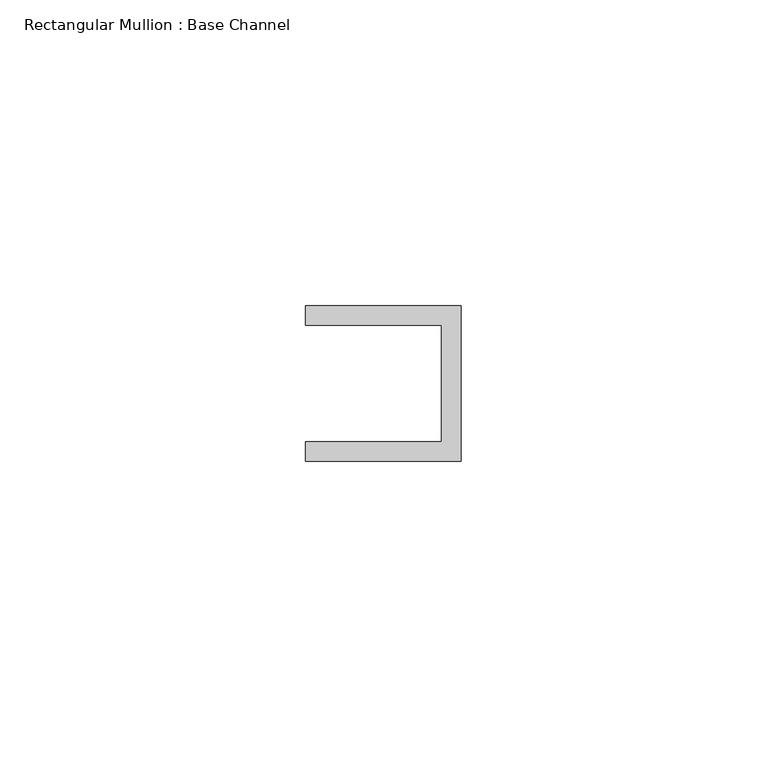
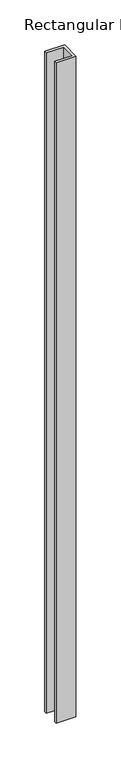
"""IFC4 building model written with IfcOpenShell, lengths in millimetres: member geometry, Rectangular Mullion : Base Channel."""

from ifc_helpers import new_model, si_unit, frame, origin, place, context, project, spatial, polyline, outline, extrude, source, transform, mapped, element, save


def rectangular_mullion_base_channel_70c3d0a8(model_context):
    return source(origin(), model_context, "Body", "SweptSolid", [
        extrude(outline(polyline([(0.0, 12.7), (0.0, -12.7), (-25.4, -12.7), (-25.4, -9.525), (-3.175, -9.525), (-3.175, 9.525), (-25.4, 9.525), (-25.4, 12.7), (0.0, 12.7)])), frame((0.0, 0.0, -898.525), z_axis=(0.0, 0.0, 1.0), x_axis=(1.0, 0.0, 0.0)), (0.0, 0.0, 1.0), 898.525),
    ])


if __name__ == "__main__":
    model = new_model("IFC4")
    model_context = context("Model", 3, world=origin())
    ifc_project = project(units=[si_unit("LENGTHUNIT", "METRE", prefix="MILLI")], contexts=[model_context])
    site = spatial("IfcSite", under=ifc_project)
    building = spatial("IfcBuilding", under=site)
    placement = place(None, origin())
    rectangular_mullion_base_channel_shape = rectangular_mullion_base_channel_70c3d0a8(model_context)
    element("IfcMember", 1, ObjectType="Rectangular Mullion : Base Channel", at=placement, inside=building, context=model_context, shape_type="MappedRepresentation", body=[
        mapped(rectangular_mullion_base_channel_shape, transform((0.0, 0.0, 0.0), x_axis=(1.0, 0.0, 0.0), y_axis=(0.0, 1.0, 0.0), z_axis=(0.0, 0.0, 1.0))),
    ])
    save(model, "model.ifc")

# Revit data of these elements
# Type "Rectangular Mullion : Base Channel"
#   built-in parameter 1007322 = 0.0833333 (stored number, unit not read)
#   built-in parameter 1007321 = 0.0416667 (stored number, unit not read)
#   built-in parameter 1007320 = -0.03125 (stored number, unit not read)
# Element 1 (IfcMember, "Rectangular Mullion : Base Channel")
#   Materials on its faces: "ALUM"
# Materials
#   "ALUM": class "Generic", colour RGB 157 157 157, transparency 0, Cost = 0
